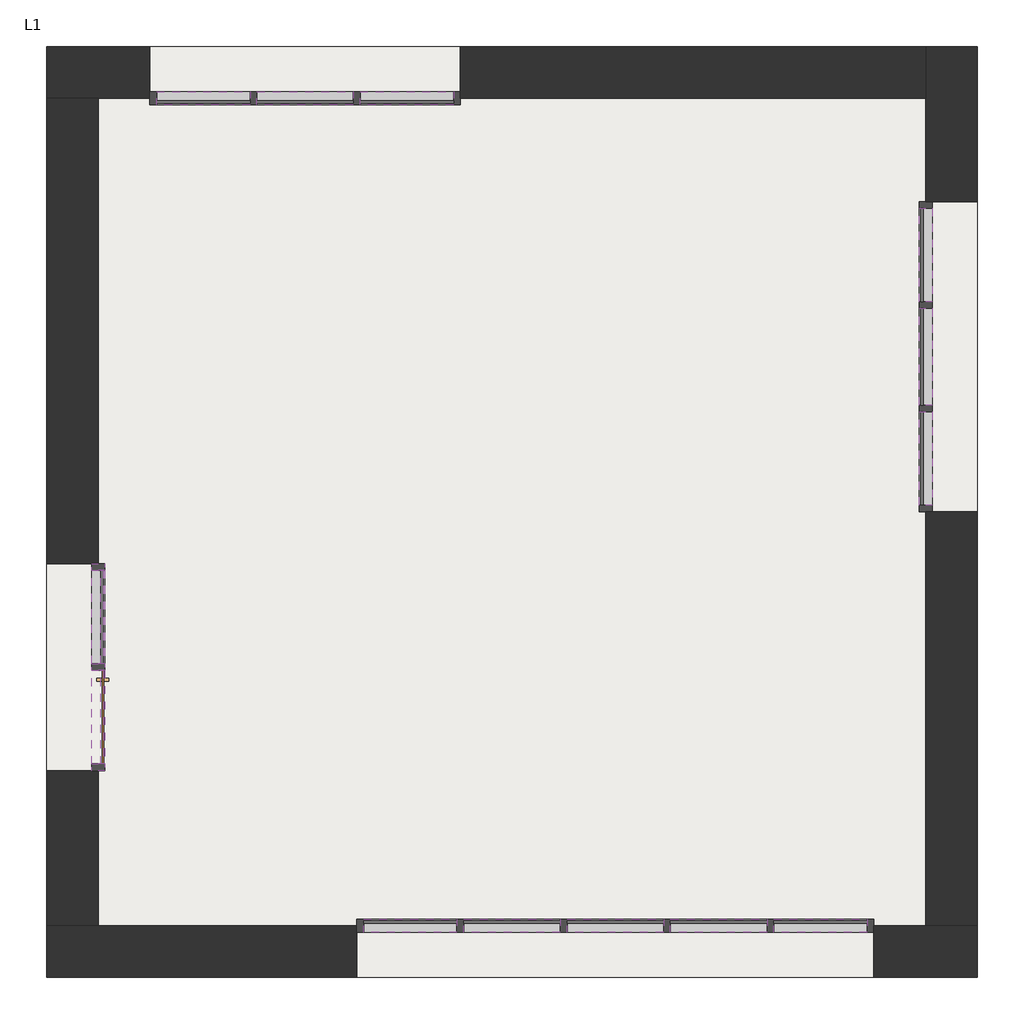
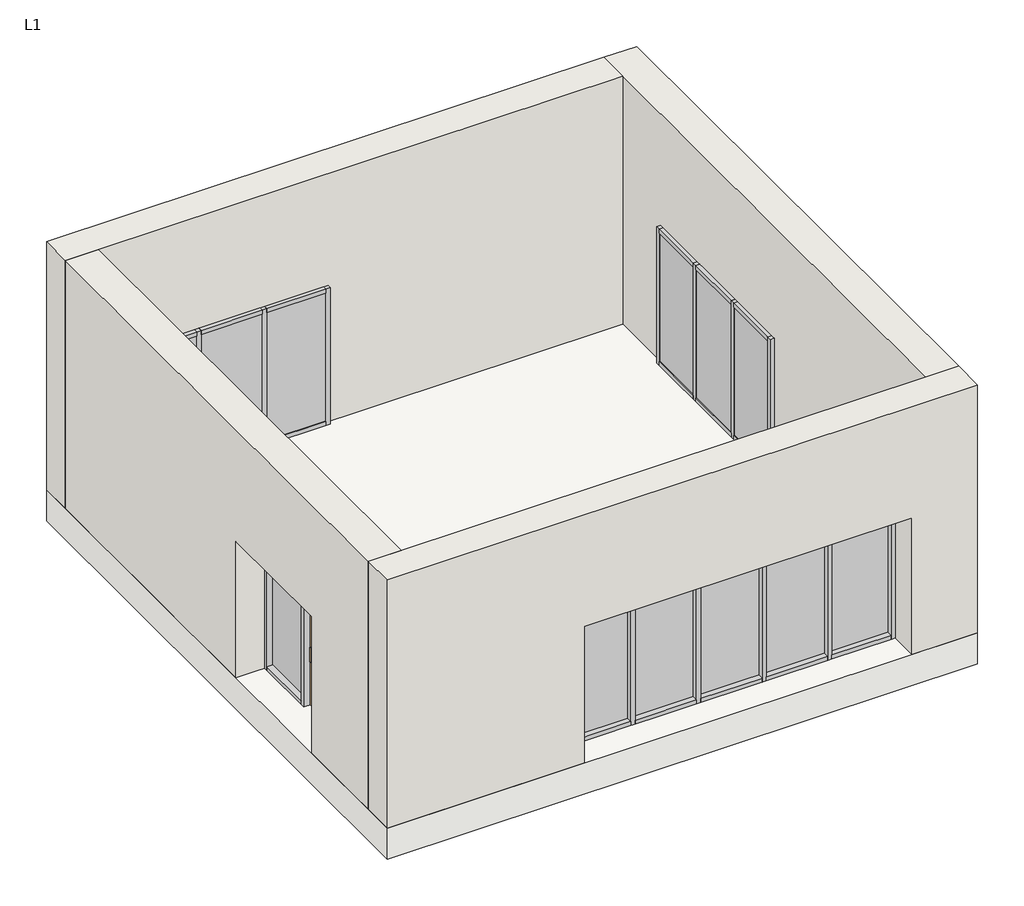
# One storey: 47 members, 14 plates, 4 walls, 1 door, 1 slab.
"""IFC4 building model written with IfcOpenShell, lengths in millimetres."""

import ifcopenshell
import ifcopenshell.guid

model = None  # the IFC model being written
_history = None  # IfcOwnerHistory: only IFC2X3 demands one
_inside = {}  # id of a spatial element -> (the spatial element, [elements in it])
_under = {}  # id of a project, library or spatial element -> (it, [spatial elements below it])
_declared = {}  # id of a project -> (the project, [libraries it declares])
_typed = {}  # id of a type object -> (the type object, [elements of that type])
_made_of = {}  # id of a material, layer set ... -> (it, [elements and type objects made of it])


def new_model(schema):
    """Start an empty IFC model of exactly this schema.

    Asked for "IFC4X3", IfcOpenShell would pick the latest addendum, in which some entities
    have other attributes; the version numbers below select the first issue.
    IFC2X3 requires an IfcOwnerHistory on every rooted entity: one is made here for all.
    """
    global model, _history
    if schema == "IFC4X3":
        model = ifcopenshell.file(schema_version=(4, 3, 0, 0))
    else:
        model = ifcopenshell.file(schema=schema)
    _inside.clear()
    _under.clear()
    _declared.clear()
    _typed.clear()
    _made_of.clear()
    _history = None
    if model.schema == "IFC2X3":
        org = make("IfcOrganization", Name="unknown")
        user = make(
            "IfcPersonAndOrganization",
            ThePerson=make("IfcPerson", FamilyName="unknown"),
            TheOrganization=org,
        )
        app = make(
            "IfcApplication",
            ApplicationDeveloper=org,
            Version="unknown",
            ApplicationFullName="unknown",
            ApplicationIdentifier="unknown",
        )
        _history = make(
            "IfcOwnerHistory",
            OwningUser=user,
            OwningApplication=app,
            ChangeAction="ADDED",
            CreationDate=0,
        )
    return model


def make(cls, **values):
    """One entity of the class cls with the attributes given. An attribute that is None is left unset."""
    return model.create_entity(
        cls, **{name: value for name, value in values.items() if value is not None}
    )


def rooted(cls, **values):
    """An entity with a GlobalId (a new one), such as an element, a storey or a relation."""
    return make(cls, GlobalId=ifcopenshell.guid.new(), OwnerHistory=_history, **values)


def si_unit(unit_type, name, prefix=None):
    """IfcSIUnit, for example si_unit("LENGTHUNIT", "METRE", prefix="MILLI")."""
    return make("IfcSIUnit", UnitType=unit_type, Prefix=prefix, Name=name)


def assignment(units):
    """IfcUnitAssignment: the units of a project."""
    return None if units is None else make("IfcUnitAssignment", Units=units)


def point(xyz):
    """IfcCartesianPoint."""
    return None if xyz is None else make("IfcCartesianPoint", Coordinates=xyz)


def direction(xyz):
    """IfcDirection."""
    return None if xyz is None else make("IfcDirection", DirectionRatios=xyz)


def frame(location, z_axis=None, x_axis=None):
    """IfcAxis2Placement3D, a coordinate frame: its origin and axes. An axis left out is left unset."""
    return make(
        "IfcAxis2Placement3D",
        Location=point(location),
        Axis=direction(z_axis),
        RefDirection=direction(x_axis),
    )


def origin():
    """The frame at (0, 0, 0) with its axes left unset."""
    return frame((0.0, 0.0, 0.0))


def origin_with_axes():
    """The frame at (0, 0, 0) with the z axis (0, 0, 1) and the x axis (1, 0, 0) written out."""
    return frame((0.0, 0.0, 0.0), z_axis=(0.0, 0.0, 1.0), x_axis=(1.0, 0.0, 0.0))


def place(relative_to, where):
    """IfcLocalPlacement: puts the frame where relative to a parent placement (None: the world)."""
    return make(
        "IfcLocalPlacement", PlacementRelTo=relative_to, RelativePlacement=where
    )


def context(
    kind, dimensions, precision=None, world=None, true_north=None, identifier=None
):
    """IfcGeometricRepresentationContext, for example the 3D "Model" context."""
    return make(
        "IfcGeometricRepresentationContext",
        ContextIdentifier=identifier,
        ContextType=kind,
        CoordinateSpaceDimension=dimensions,
        Precision=precision,
        WorldCoordinateSystem=world,
        TrueNorth=true_north,
    )


def project(units=None, contexts=None):
    """IfcProject with its units and contexts."""
    return rooted(
        "IfcProject",
        Name="project",
        RepresentationContexts=contexts,
        UnitsInContext=assignment(units),
    )


def spatial(cls, under=None, at=None, **own):
    """A site, building, storey or space (cls), placed at a placement, below another one or the project."""
    s = rooted(cls, ObjectPlacement=at, **own)
    if under is not None:
        _under.setdefault(under.id(), (under, []))[1].append(s)
    return s


def polyline(points):
    """IfcPolyline through the points."""
    return make("IfcPolyline", Points=[point(p) for p in points])


def outline(outer, holes=None, kind="AREA"):
    """IfcArbitraryClosedProfileDef: a profile drawn as a closed curve; with holes, ...WithVoids."""
    if holes is None:
        return make("IfcArbitraryClosedProfileDef", ProfileType=kind, OuterCurve=outer)
    return make(
        "IfcArbitraryProfileDefWithVoids",
        ProfileType=kind,
        OuterCurve=outer,
        InnerCurves=holes,
    )


def extrude(swept, where, along, depth):
    """IfcExtrudedAreaSolid: the profile swept, set in the frame where, extruded along a direction by depth."""
    return make(
        "IfcExtrudedAreaSolid",
        SweptArea=swept,
        Position=where,
        ExtrudedDirection=direction(along),
        Depth=depth,
    )


def faces_of(points, faces, orient=None, outer=None):
    """IfcFace entities. A face is a list of loops; a loop is a list of indices into points, from 0.

    orient and outer hold one flag for each loop. By default every Orientation is true, the
    first loop of a face is its IfcFaceOuterBound and the others are IfcFaceBound.
    """
    made = []
    for i, loops in enumerate(faces):
        bounds = []
        for j, loop in enumerate(loops):
            is_outer = j == 0 if outer is None else outer[i][j]
            bounds.append(
                make(
                    "IfcFaceOuterBound" if is_outer else "IfcFaceBound",
                    Bound=make("IfcPolyLoop", Polygon=[points[k] for k in loop]),
                    Orientation=True if orient is None else orient[i][j],
                )
            )
        made.append(make("IfcFace", Bounds=bounds))
    return made


def faceted_brep(points, faces, orient=None, outer=None, voids=None):
    """IfcFacetedBrep: a solid bounded by flat faces; with voids (closed shells), ...WithVoids."""
    shared = [point(p) for p in points]
    hull = make("IfcClosedShell", CfsFaces=faces_of(shared, faces, orient, outer))
    if voids is None:
        return make("IfcFacetedBrep", Outer=hull)
    return make(
        "IfcFacetedBrepWithVoids",
        Outer=hull,
        Voids=[
            make(cls, CfsFaces=faces_of(shared, fs, o, b)) for cls, fs, o, b in voids
        ],
    )


def shape(context_of_items, identifier, shape_type, items):
    """IfcShapeRepresentation: the items that make up one representation, for example the "Body"."""
    return make(
        "IfcShapeRepresentation",
        ContextOfItems=context_of_items,
        RepresentationIdentifier=identifier,
        RepresentationType=shape_type,
        Items=items,
    )


def source(mapping_origin, context_of_items, identifier, shape_type, items):
    """IfcRepresentationMap: a shape defined once, which mapped items show again and again."""
    return make(
        "IfcRepresentationMap",
        MappingOrigin=mapping_origin,
        MappedRepresentation=shape(context_of_items, identifier, shape_type, items),
    )


def transform(
    local_origin,
    x_axis=None,
    y_axis=None,
    z_axis=None,
    scale=None,
    scale2=None,
    scale3=None,
    uniform=True,
):
    """IfcCartesianTransformationOperator3D, or its non-uniform kind. x_axis, y_axis, z_axis: its Axis1, 2, 3."""
    if uniform:
        return make(
            "IfcCartesianTransformationOperator3D",
            Axis1=direction(x_axis),
            Axis2=direction(y_axis),
            LocalOrigin=point(local_origin),
            Scale=scale,
            Axis3=direction(z_axis),
        )
    return make(
        "IfcCartesianTransformationOperator3DnonUniform",
        Axis1=direction(x_axis),
        Axis2=direction(y_axis),
        LocalOrigin=point(local_origin),
        Scale=scale,
        Axis3=direction(z_axis),
        Scale2=scale2,
        Scale3=scale3,
    )


def mapped(mapping_source, mapping_target):
    """IfcMappedItem: shows the shape of a source again, moved by a transform."""
    return make(
        "IfcMappedItem", MappingSource=mapping_source, MappingTarget=mapping_target
    )


def made_of(thing, what):
    """Note that an element or type object is made of a material, layer set ...; save() writes the relation."""
    if what is not None:
        _made_of.setdefault(what.id(), (what, []))[1].append(thing)
    return thing


def element(
    cls,
    number,
    at=None,
    inside=None,
    cuts=None,
    type_object=None,
    material=None,
    context=None,
    identifier="Body",
    shape_type=None,
    held_by="IfcProductDefinitionShape",
    body=None,
    shapes=None,
    **own,
):
    """One element of the class cls, such as IfcWall. Its Tag is "e" and its number.

    at: its placement. inside: the storey or other place that contains it. cuts: it is an
    opening in that element (IfcRelVoidsElement). A single representation is given by context,
    identifier, shape_type and body (its items); several are given by shapes. held_by: the class
    of the entity that holds the representations. save() writes the other relations.
    """
    e = rooted(cls, Tag="e%d" % number, ObjectPlacement=at, **own)
    if body is not None:
        shapes = [shape(context, identifier, shape_type, body)]
    if shapes is not None:
        e.Representation = make(held_by, Representations=shapes)
    if inside is not None:
        _inside.setdefault(inside.id(), (inside, []))[1].append(e)
    if cuts is not None:
        rooted(
            "IfcRelVoidsElement", RelatingBuildingElement=cuts, RelatedOpeningElement=e
        )
    if type_object is not None:
        _typed.setdefault(type_object.id(), (type_object, []))[1].append(e)
    return made_of(e, material)


def aggregate(whole, parts):
    """IfcRelAggregates: a whole, such as a stair, and the parts it consists of."""
    return rooted("IfcRelAggregates", RelatingObject=whole, RelatedObjects=parts)


def save(model, path):
    """Write the relations noted so far, then the file.

    IfcRelAggregates (storeys below a building ...), IfcRelContainedInSpatialStructure (elements
    in a storey), IfcRelDefinesByType, IfcRelAssociatesMaterial and IfcRelDeclares: one each for
    every whole, place, type object, material and project.
    """
    for whole, parts in _under.values():
        aggregate(whole, parts)
    for where, things in _inside.values():
        rooted(
            "IfcRelContainedInSpatialStructure",
            RelatedElements=things,
            RelatingStructure=where,
        )
    for kind, things in _typed.values():
        rooted("IfcRelDefinesByType", RelatedObjects=things, RelatingType=kind)
    for what, things in _made_of.values():
        rooted("IfcRelAssociatesMaterial", RelatedObjects=things, RelatingMaterial=what)
    for by, libraries in _declared.values():
        rooted("IfcRelDeclares", RelatingContext=by, RelatedDefinitions=libraries)
    model.write(path)


def m_door_curtain_wall_single_glass_m_door_curtain_wall_single_b3f25844(model_context):
    return source(origin(), model_context, "Body", "SweptSolid", [
        extrude(outline(polyline([(451.2499998, 50.8), (451.2499998, 38.1), (-451.2499998, 38.1), (-451.2499998, 50.8), (451.2499998, 50.8)])), origin_with_axes(), (0.0, 0.0, 1.0), 1967.5),
        extrude(outline(polyline([(-375.0499998, 101.6), (-349.6499998, 101.6), (-349.6499998, 50.8), (-375.0499998, 50.8), (-375.0499998, 101.6)])), frame((0.0, 0.0, 762.0), z_axis=(0.0, 0.0, 1.0), x_axis=(1.0, 0.0, 0.0)), (0.0, 0.0, 1.0), 228.6),
        extrude(outline(polyline([(-349.6499998, -12.7), (-375.0499998, -12.7), (-375.0499998, 38.1), (-349.6499998, 38.1), (-349.6499998, -12.7)])), frame((0.0, 0.0, 762.0), z_axis=(0.0, 0.0, 1.0), x_axis=(1.0, 0.0, 0.0)), (0.0, 0.0, 1.0), 228.6),
    ])


def rectangular_mullion_65_x_125mm_rectangular_3ebb1efe(model_context):
    return source(origin(), model_context, "Body", "SweptSolid", [
        extrude(outline(polyline([(32.5, 62.5), (32.5, -62.5), (-32.5, -62.5), (-32.5, 62.5), (32.5, 62.5)])), frame((0.0, 0.0, -2200.0), z_axis=(0.0, 0.0, 1.0), x_axis=(1.0, 0.0, 0.0)), (0.0, 0.0, 1.0), 2200.0),
    ])


def rectangular_mullion_65_x_125mm_rectangular_02dc2359(model_context):
    return source(origin(), model_context, "Body", "SweptSolid", [
        extrude(outline(polyline([(0.0, 62.5), (0.0, -62.5), (-65.0, -62.5), (-65.0, 62.5), (0.0, 62.5)])), frame((0.0, 0.0, -2200.0), z_axis=(0.0, 0.0, 1.0), x_axis=(1.0, 0.0, 0.0)), (0.0, 0.0, 1.0), 2200.0),
    ])


def rectangular_mullion_65_x_125mm_rectangular_9a77bebc(model_context):
    return source(origin(), model_context, "Body", "SweptSolid", [
        extrude(outline(polyline([(0.0, 62.5), (0.0, -62.5), (-65.0, -62.5), (-65.0, 62.5), (0.0, 62.5)])), frame((0.0, 0.0, -902.5000003), z_axis=(0.0, 0.0, 1.0), x_axis=(1.0, 0.0, 0.0)), (0.0, 0.0, 1.0), 902.5000003),
    ])


def rectangular_mullion_65_x_125mm_rectangular_1b57746c(model_context):
    return source(origin(), model_context, "Body", "SweptSolid", [
        extrude(outline(polyline([(0.0, 62.5), (0.0, -62.5), (-65.0, -62.5), (-65.0, 62.5), (0.0, 62.5)])), frame((0.0, 0.0, -935.0), z_axis=(0.0, 0.0, 1.0), x_axis=(1.0, 0.0, 0.0)), (0.0, 0.0, 1.0), 935.0),
    ])


def rectangular_mullion_65_x_125mm_rectangular_ad388592(model_context):
    return source(origin(), model_context, "Body", "SweptSolid", [
        extrude(outline(polyline([(32.5, 62.5), (32.5, -62.5), (-32.5, -62.5), (-32.5, 62.5), (32.5, 62.5)])), frame((0.0, 0.0, -902.5000003), z_axis=(0.0, 0.0, 1.0), x_axis=(1.0, 0.0, 0.0)), (0.0, 0.0, 1.0), 902.5000003),
    ])


def rectangular_mullion_65_x_125mm_rectangular_470365d3(model_context):
    return source(origin(), model_context, "Body", "SweptSolid", [
        extrude(outline(polyline([(32.5, 62.5), (32.5, -62.5), (-32.5, -62.5), (-32.5, 62.5), (32.5, 62.5)])), frame((0.0, 0.0, -200.0), z_axis=(0.0, 0.0, 1.0), x_axis=(1.0, 0.0, 0.0)), (0.0, 0.0, 1.0), 200.0),
    ])


def rectangular_mullion_65_x_125mm_rectangular_dd0f1ba9(model_context):
    return source(origin(), model_context, "Body", "SweptSolid", [
        extrude(outline(polyline([(0.0, 62.5), (0.0, -62.5), (-65.0, -62.5), (-65.0, 62.5), (0.0, 62.5)])), frame((0.0, 0.0, -200.0), z_axis=(0.0, 0.0, 1.0), x_axis=(1.0, 0.0, 0.0)), (0.0, 0.0, 1.0), 200.0),
    ])


def rectangular_mullion_65_x_125mm_rectangular_b62c991d(model_context):
    return source(origin(), model_context, "Body", "SweptSolid", [
        extrude(outline(polyline([(32.5, 62.5), (32.5, -62.5), (-32.5, -62.5), (-32.5, 62.5), (32.5, 62.5)])), frame((0.0, 0.0, -2000.0), z_axis=(0.0, 0.0, 1.0), x_axis=(1.0, 0.0, 0.0)), (0.0, 0.0, 1.0), 2000.0),
    ])


def rectangular_mullion_65_x_125mm_rectangular_d57ab73f(model_context):
    return source(origin(), model_context, "Body", "SweptSolid", [
        extrude(outline(polyline([(0.0, 62.5), (0.0, -62.5), (-65.0, -62.5), (-65.0, 62.5), (0.0, 62.5)])), frame((0.0, 0.0, -2000.0), z_axis=(0.0, 0.0, 1.0), x_axis=(1.0, 0.0, 0.0)), (0.0, 0.0, 1.0), 2000.0),
    ])


def system_panel_glazed_3f8cfcef(model_context):
    return source(origin(), model_context, "Body", "SweptSolid", [
        extrude(outline(polyline([(451.2500002, 24.5), (-451.2500002, 24.5), (-451.2500002, 49.5), (451.2500002, 49.5), (451.2500002, 24.5)])), origin_with_axes(), (0.0, 0.0, 1.0), 2070.0),
    ])


def system_panel_glazed_4c7b465e(model_context):
    return source(origin(), model_context, "Body", "SweptSolid", [
        extrude(outline(polyline([(467.5, 24.5), (-467.5, 24.5), (-467.5, 49.5), (467.5, 49.5), (467.5, 24.5)])), origin_with_axes(), (0.0, 0.0, 1.0), 2070.0),
    ])


def system_panel_glazed_7330a8e7(model_context):
    return source(origin(), model_context, "Body", "SweptSolid", [
        extrude(outline(polyline([(451.2500002, 24.5), (-451.2500002, 24.5), (-451.2500002, 49.5), (451.2500002, 49.5), (451.2500002, 24.5)])), origin_with_axes(), (0.0, 0.0, 1.0), 102.5),
    ])


def system_panel_glazed_53f32d20(model_context):
    return source(origin(), model_context, "Body", "SweptSolid", [
        extrude(outline(polyline([(451.2500002, 24.5), (-451.2500002, 24.5), (-451.2500002, 49.5), (451.2500002, 49.5), (451.2500002, 24.5)])), origin_with_axes(), (0.0, 0.0, 1.0), 1902.5),
    ])


model = new_model("IFC4")

# Units and contexts
model_context = context("Model", 3, world=origin())
ifc_project = project(units=[si_unit("LENGTHUNIT", "METRE", prefix="MILLI")], contexts=[model_context])

# Site, building, storey
site = spatial("IfcSite", under=ifc_project)
building = spatial("IfcBuilding", under=site)
storey = spatial("IfcBuildingStorey", under=building, Name="L1", Elevation=0.0)

# Door
placement = place(None, origin())
m_door_curtain_wall_single_glass_m_door_curtain_wall_single_shape = m_door_curtain_wall_single_glass_m_door_curtain_wall_single_b3f25844(model_context)
element("IfcDoor", 1, ObjectType="M_Door-Curtain-Wall-Single-Glass : M_Door-Curtain-Wall-Single-Glass", at=placement, inside=storey, context=model_context, shape_type="MappedRepresentation", body=[
    mapped(m_door_curtain_wall_single_glass_m_door_curtain_wall_single_shape, transform((500.000016, 1516.2441438, 0.0), x_axis=(0.0, -1.0, 0.0), y_axis=(1.0, 0.0, 0.0), z_axis=(0.0, 0.0, 1.0))),
])

# Members
rectangular_mullion_65_x_125mm_rectangular_shape = rectangular_mullion_65_x_125mm_rectangular_3ebb1efe(model_context)
element("IfcMember", 2, ObjectType="Rectangular Mullion : 65 x 125mm rectangular", at=placement, inside=storey, context=model_context, shape_type="MappedRepresentation", body=[
    mapped(rectangular_mullion_65_x_125mm_rectangular_shape, transform((4000.0000163, -500.0058491, 0.0), x_axis=(1.0, 0.0, 0.0), y_axis=(0.0, -1.0, 0.0), z_axis=(0.0, 0.0, -1.0))),
])
element("IfcMember", 3, ObjectType="Rectangular Mullion : 65 x 125mm rectangular", at=placement, inside=storey, context=model_context, shape_type="MappedRepresentation", body=[
    mapped(rectangular_mullion_65_x_125mm_rectangular_shape, transform((5000.0000163, -500.0058491, 0.0), x_axis=(1.0, 0.0, 0.0), y_axis=(0.0, -1.0, 0.0), z_axis=(0.0, 0.0, -1.0))),
])
element("IfcMember", 4, ObjectType="Rectangular Mullion : 65 x 125mm rectangular", at=placement, inside=storey, context=model_context, shape_type="MappedRepresentation", body=[
    mapped(rectangular_mullion_65_x_125mm_rectangular_shape, transform((6000.0000163, -500.0058491, 0.0), x_axis=(1.0, 0.0, 0.0), y_axis=(0.0, -1.0, 0.0), z_axis=(0.0, 0.0, -1.0))),
])
element("IfcMember", 5, ObjectType="Rectangular Mullion : 65 x 125mm rectangular", at=placement, inside=storey, context=model_context, shape_type="MappedRepresentation", body=[
    mapped(rectangular_mullion_65_x_125mm_rectangular_shape, transform((7000.0000163, -500.0058491, 0.0), x_axis=(1.0, 0.0, 0.0), y_axis=(0.0, -1.0, 0.0), z_axis=(0.0, 0.0, -1.0))),
])
element("IfcMember", 6, ObjectType="Rectangular Mullion : 65 x 125mm rectangular", at=placement, inside=storey, context=model_context, shape_type="MappedRepresentation", body=[
    mapped(rectangular_mullion_65_x_125mm_rectangular_shape, transform((8500.000016, 4499.9941443, 0.0), x_axis=(0.0, 1.0, 0.0), y_axis=(1.0, 0.0, 0.0), z_axis=(0.0, 0.0, -1.0))),
])
element("IfcMember", 7, ObjectType="Rectangular Mullion : 65 x 125mm rectangular", at=placement, inside=storey, context=model_context, shape_type="MappedRepresentation", body=[
    mapped(rectangular_mullion_65_x_125mm_rectangular_shape, transform((8500.000016, 5499.9941443, 0.0), x_axis=(0.0, 1.0, 0.0), y_axis=(1.0, 0.0, 0.0), z_axis=(0.0, 0.0, -1.0))),
])
element("IfcMember", 8, ObjectType="Rectangular Mullion : 65 x 125mm rectangular", at=placement, inside=storey, context=model_context, shape_type="MappedRepresentation", body=[
    mapped(rectangular_mullion_65_x_125mm_rectangular_shape, transform((3000.0000157, 7499.994144, 0.0), x_axis=(-1.0, 0.0, 0.0), y_axis=(0.0, 1.0, 0.0), z_axis=(0.0, 0.0, -1.0))),
])
element("IfcMember", 9, ObjectType="Rectangular Mullion : 65 x 125mm rectangular", at=placement, inside=storey, context=model_context, shape_type="MappedRepresentation", body=[
    mapped(rectangular_mullion_65_x_125mm_rectangular_shape, transform((2000.0000157, 7499.994144, 0.0), x_axis=(-1.0, 0.0, 0.0), y_axis=(0.0, 1.0, 0.0), z_axis=(0.0, 0.0, -1.0))),
])
rectangular_mullion_65_x_125mm_rectangular_2_shape = rectangular_mullion_65_x_125mm_rectangular_02dc2359(model_context)
element("IfcMember", 10, ObjectType="Rectangular Mullion : 65 x 125mm rectangular", at=placement, inside=storey, context=model_context, shape_type="MappedRepresentation", body=[
    mapped(rectangular_mullion_65_x_125mm_rectangular_2_shape, transform((8000.000016, -500.0058491, 0.0), x_axis=(1.0, 0.0, 0.0), y_axis=(0.0, -1.0, 0.0), z_axis=(0.0, 0.0, -1.0))),
])
element("IfcMember", 11, ObjectType="Rectangular Mullion : 65 x 125mm rectangular", at=placement, inside=storey, context=model_context, shape_type="MappedRepresentation", body=[
    mapped(rectangular_mullion_65_x_125mm_rectangular_2_shape, transform((8500.000016, 6499.994144, 0.0), x_axis=(0.0, 1.0, 0.0), y_axis=(1.0, 0.0, 0.0), z_axis=(0.0, 0.0, -1.0))),
])
element("IfcMember", 12, ObjectType="Rectangular Mullion : 65 x 125mm rectangular", at=placement, inside=storey, context=model_context, shape_type="MappedRepresentation", body=[
    mapped(rectangular_mullion_65_x_125mm_rectangular_2_shape, transform((1000.000016, 7499.994144, 0.0), x_axis=(-1.0, 0.0, 0.0), y_axis=(0.0, 1.0, 0.0), z_axis=(0.0, 0.0, -1.0))),
])
element("IfcMember", 13, ObjectType="Rectangular Mullion : 65 x 125mm rectangular", at=placement, inside=storey, context=model_context, shape_type="MappedRepresentation", body=[
    mapped(rectangular_mullion_65_x_125mm_rectangular_2_shape, transform((3000.000016, -500.0058491, 2200.0), x_axis=(-1.0, 0.0, 0.0), y_axis=(0.0, -1.0, 0.0), z_axis=(0.0, 0.0, 1.0))),
])
element("IfcMember", 14, ObjectType="Rectangular Mullion : 65 x 125mm rectangular", at=placement, inside=storey, context=model_context, shape_type="MappedRepresentation", body=[
    mapped(rectangular_mullion_65_x_125mm_rectangular_2_shape, transform((8500.000016, 3499.994144, 2200.0), x_axis=(0.0, -1.0, 0.0), y_axis=(1.0, 0.0, 0.0), z_axis=(0.0, 0.0, 1.0))),
])
element("IfcMember", 15, ObjectType="Rectangular Mullion : 65 x 125mm rectangular", at=placement, inside=storey, context=model_context, shape_type="MappedRepresentation", body=[
    mapped(rectangular_mullion_65_x_125mm_rectangular_2_shape, transform((4000.000016, 7499.994144, 2200.0), x_axis=(1.0, 0.0, 0.0), y_axis=(0.0, 1.0, 0.0), z_axis=(0.0, 0.0, 1.0))),
])
rectangular_mullion_65_x_125mm_rectangular_3_shape = rectangular_mullion_65_x_125mm_rectangular_9a77bebc(model_context)
element("IfcMember", 16, ObjectType="Rectangular Mullion : 65 x 125mm rectangular", at=placement, inside=storey, context=model_context, shape_type="MappedRepresentation", body=[
    mapped(rectangular_mullion_65_x_125mm_rectangular_3_shape, transform((7935.000016, -500.0058491, 2200.0), x_axis=(0.0, 0.0, 1.0), y_axis=(0.0, -1.0, 0.0), z_axis=(1.0, 0.0, 0.0))),
])
element("IfcMember", 17, ObjectType="Rectangular Mullion : 65 x 125mm rectangular", at=placement, inside=storey, context=model_context, shape_type="MappedRepresentation", body=[
    mapped(rectangular_mullion_65_x_125mm_rectangular_3_shape, transform((3967.5000163, -500.0058491, 2200.0), x_axis=(0.0, 0.0, 1.0), y_axis=(0.0, -1.0, 0.0), z_axis=(1.0, 0.0, 0.0))),
])
element("IfcMember", 18, ObjectType="Rectangular Mullion : 65 x 125mm rectangular", at=placement, inside=storey, context=model_context, shape_type="MappedRepresentation", body=[
    mapped(rectangular_mullion_65_x_125mm_rectangular_3_shape, transform((8500.000016, 6434.994144, 2200.0), x_axis=(0.0, 0.0, 1.0), y_axis=(1.0, 0.0, 0.0), z_axis=(0.0, 1.0, 0.0))),
])
element("IfcMember", 19, ObjectType="Rectangular Mullion : 65 x 125mm rectangular", at=placement, inside=storey, context=model_context, shape_type="MappedRepresentation", body=[
    mapped(rectangular_mullion_65_x_125mm_rectangular_3_shape, transform((8500.000016, 4467.4941443, 2200.0), x_axis=(0.0, 0.0, 1.0), y_axis=(1.0, 0.0, 0.0), z_axis=(0.0, 1.0, 0.0))),
])
element("IfcMember", 20, ObjectType="Rectangular Mullion : 65 x 125mm rectangular", at=placement, inside=storey, context=model_context, shape_type="MappedRepresentation", body=[
    mapped(rectangular_mullion_65_x_125mm_rectangular_3_shape, transform((1065.000016, 7499.994144, 2200.0), x_axis=(0.0, 0.0, 1.0), y_axis=(0.0, 1.0, 0.0), z_axis=(-1.0, 0.0, 0.0))),
])
element("IfcMember", 21, ObjectType="Rectangular Mullion : 65 x 125mm rectangular", at=placement, inside=storey, context=model_context, shape_type="MappedRepresentation", body=[
    mapped(rectangular_mullion_65_x_125mm_rectangular_3_shape, transform((3032.5000157, 7499.994144, 2200.0), x_axis=(0.0, 0.0, 1.0), y_axis=(0.0, 1.0, 0.0), z_axis=(-1.0, 0.0, 0.0))),
])
element("IfcMember", 22, ObjectType="Rectangular Mullion : 65 x 125mm rectangular", at=placement, inside=storey, context=model_context, shape_type="MappedRepresentation", body=[
    mapped(rectangular_mullion_65_x_125mm_rectangular_3_shape, transform((500.000016, 1064.994144, 2200.0), x_axis=(0.0, 0.0, 1.0), y_axis=(-1.0, 0.0, 0.0), z_axis=(0.0, -1.0, 0.0))),
])
element("IfcMember", 23, ObjectType="Rectangular Mullion : 65 x 125mm rectangular", at=placement, inside=storey, context=model_context, shape_type="MappedRepresentation", body=[
    mapped(rectangular_mullion_65_x_125mm_rectangular_3_shape, transform((500.000016, 2032.4941437, 2200.0), x_axis=(0.0, 0.0, 1.0), y_axis=(-1.0, 0.0, 0.0), z_axis=(0.0, -1.0, 0.0))),
])
rectangular_mullion_65_x_125mm_rectangular_4_shape = rectangular_mullion_65_x_125mm_rectangular_1b57746c(model_context)
element("IfcMember", 24, ObjectType="Rectangular Mullion : 65 x 125mm rectangular", at=placement, inside=storey, context=model_context, shape_type="MappedRepresentation", body=[
    mapped(rectangular_mullion_65_x_125mm_rectangular_4_shape, transform((4967.5000163, -500.0058491, 2200.0), x_axis=(0.0, 0.0, 1.0), y_axis=(0.0, -1.0, 0.0), z_axis=(1.0, 0.0, 0.0))),
])
element("IfcMember", 25, ObjectType="Rectangular Mullion : 65 x 125mm rectangular", at=placement, inside=storey, context=model_context, shape_type="MappedRepresentation", body=[
    mapped(rectangular_mullion_65_x_125mm_rectangular_4_shape, transform((5967.5000163, -500.0058491, 2200.0), x_axis=(0.0, 0.0, 1.0), y_axis=(0.0, -1.0, 0.0), z_axis=(1.0, 0.0, 0.0))),
])
element("IfcMember", 26, ObjectType="Rectangular Mullion : 65 x 125mm rectangular", at=placement, inside=storey, context=model_context, shape_type="MappedRepresentation", body=[
    mapped(rectangular_mullion_65_x_125mm_rectangular_4_shape, transform((6967.5000163, -500.0058491, 2200.0), x_axis=(0.0, 0.0, 1.0), y_axis=(0.0, -1.0, 0.0), z_axis=(1.0, 0.0, 0.0))),
])
element("IfcMember", 27, ObjectType="Rectangular Mullion : 65 x 125mm rectangular", at=placement, inside=storey, context=model_context, shape_type="MappedRepresentation", body=[
    mapped(rectangular_mullion_65_x_125mm_rectangular_4_shape, transform((8500.000016, 5467.4941443, 2200.0), x_axis=(0.0, 0.0, 1.0), y_axis=(1.0, 0.0, 0.0), z_axis=(0.0, 1.0, 0.0))),
])
element("IfcMember", 28, ObjectType="Rectangular Mullion : 65 x 125mm rectangular", at=placement, inside=storey, context=model_context, shape_type="MappedRepresentation", body=[
    mapped(rectangular_mullion_65_x_125mm_rectangular_4_shape, transform((2032.5000157, 7499.994144, 2200.0), x_axis=(0.0, 0.0, 1.0), y_axis=(0.0, 1.0, 0.0), z_axis=(-1.0, 0.0, 0.0))),
])
element("IfcMember", 29, ObjectType="Rectangular Mullion : 65 x 125mm rectangular", at=placement, inside=storey, context=model_context, shape_type="MappedRepresentation", body=[
    mapped(rectangular_mullion_65_x_125mm_rectangular_3_shape, transform((3065.000016, -500.0058491, 0.0), x_axis=(0.0, 0.0, -1.0), y_axis=(0.0, -1.0, 0.0), z_axis=(-1.0, 0.0, 0.0))),
])
element("IfcMember", 30, ObjectType="Rectangular Mullion : 65 x 125mm rectangular", at=placement, inside=storey, context=model_context, shape_type="MappedRepresentation", body=[
    mapped(rectangular_mullion_65_x_125mm_rectangular_3_shape, transform((7032.5000163, -500.0058491, 0.0), x_axis=(0.0, 0.0, -1.0), y_axis=(0.0, -1.0, 0.0), z_axis=(-1.0, 0.0, 0.0))),
])
element("IfcMember", 31, ObjectType="Rectangular Mullion : 65 x 125mm rectangular", at=placement, inside=storey, context=model_context, shape_type="MappedRepresentation", body=[
    mapped(rectangular_mullion_65_x_125mm_rectangular_3_shape, transform((8500.000016, 3564.994144, 0.0), x_axis=(0.0, 0.0, -1.0), y_axis=(1.0, 0.0, 0.0), z_axis=(0.0, -1.0, 0.0))),
])
element("IfcMember", 32, ObjectType="Rectangular Mullion : 65 x 125mm rectangular", at=placement, inside=storey, context=model_context, shape_type="MappedRepresentation", body=[
    mapped(rectangular_mullion_65_x_125mm_rectangular_3_shape, transform((8500.000016, 5532.4941443, 0.0), x_axis=(0.0, 0.0, -1.0), y_axis=(1.0, 0.0, 0.0), z_axis=(0.0, -1.0, 0.0))),
])
element("IfcMember", 33, ObjectType="Rectangular Mullion : 65 x 125mm rectangular", at=placement, inside=storey, context=model_context, shape_type="MappedRepresentation", body=[
    mapped(rectangular_mullion_65_x_125mm_rectangular_3_shape, transform((3935.000016, 7499.994144, 0.0), x_axis=(0.0, 0.0, -1.0), y_axis=(0.0, 1.0, 0.0), z_axis=(1.0, 0.0, 0.0))),
])
element("IfcMember", 34, ObjectType="Rectangular Mullion : 65 x 125mm rectangular", at=placement, inside=storey, context=model_context, shape_type="MappedRepresentation", body=[
    mapped(rectangular_mullion_65_x_125mm_rectangular_3_shape, transform((1967.5000157, 7499.994144, 0.0), x_axis=(0.0, 0.0, -1.0), y_axis=(0.0, 1.0, 0.0), z_axis=(1.0, 0.0, 0.0))),
])
element("IfcMember", 35, ObjectType="Rectangular Mullion : 65 x 125mm rectangular", at=placement, inside=storey, context=model_context, shape_type="MappedRepresentation", body=[
    mapped(rectangular_mullion_65_x_125mm_rectangular_3_shape, transform((500.000016, 2934.994144, 0.0), x_axis=(0.0, 0.0, -1.0), y_axis=(-1.0, 0.0, 0.0), z_axis=(0.0, 1.0, 0.0))),
])
element("IfcMember", 36, ObjectType="Rectangular Mullion : 65 x 125mm rectangular", at=placement, inside=storey, context=model_context, shape_type="MappedRepresentation", body=[
    mapped(rectangular_mullion_65_x_125mm_rectangular_4_shape, transform((4032.5000163, -500.0058491, 0.0), x_axis=(0.0, 0.0, -1.0), y_axis=(0.0, -1.0, 0.0), z_axis=(-1.0, 0.0, 0.0))),
])
element("IfcMember", 37, ObjectType="Rectangular Mullion : 65 x 125mm rectangular", at=placement, inside=storey, context=model_context, shape_type="MappedRepresentation", body=[
    mapped(rectangular_mullion_65_x_125mm_rectangular_4_shape, transform((5032.5000163, -500.0058491, 0.0), x_axis=(0.0, 0.0, -1.0), y_axis=(0.0, -1.0, 0.0), z_axis=(-1.0, 0.0, 0.0))),
])
element("IfcMember", 38, ObjectType="Rectangular Mullion : 65 x 125mm rectangular", at=placement, inside=storey, context=model_context, shape_type="MappedRepresentation", body=[
    mapped(rectangular_mullion_65_x_125mm_rectangular_4_shape, transform((6032.5000163, -500.0058491, 0.0), x_axis=(0.0, 0.0, -1.0), y_axis=(0.0, -1.0, 0.0), z_axis=(-1.0, 0.0, 0.0))),
])
element("IfcMember", 39, ObjectType="Rectangular Mullion : 65 x 125mm rectangular", at=placement, inside=storey, context=model_context, shape_type="MappedRepresentation", body=[
    mapped(rectangular_mullion_65_x_125mm_rectangular_4_shape, transform((8500.000016, 4532.4941443, 0.0), x_axis=(0.0, 0.0, -1.0), y_axis=(1.0, 0.0, 0.0), z_axis=(0.0, -1.0, 0.0))),
])
element("IfcMember", 40, ObjectType="Rectangular Mullion : 65 x 125mm rectangular", at=placement, inside=storey, context=model_context, shape_type="MappedRepresentation", body=[
    mapped(rectangular_mullion_65_x_125mm_rectangular_4_shape, transform((2967.5000157, 7499.994144, 0.0), x_axis=(0.0, 0.0, -1.0), y_axis=(0.0, 1.0, 0.0), z_axis=(1.0, 0.0, 0.0))),
])
rectangular_mullion_65_x_125mm_rectangular_5_shape = rectangular_mullion_65_x_125mm_rectangular_ad388592(model_context)
element("IfcMember", 41, ObjectType="Rectangular Mullion : 65 x 125mm rectangular", at=placement, inside=storey, context=model_context, shape_type="MappedRepresentation", body=[
    mapped(rectangular_mullion_65_x_125mm_rectangular_5_shape, transform((500.000016, 2032.4941437, 2000.0), x_axis=(0.0, 0.0, 1.0), y_axis=(-1.0, 0.0, 0.0), z_axis=(0.0, -1.0, 0.0))),
])
element("IfcMember", 42, ObjectType="Rectangular Mullion : 65 x 125mm rectangular", at=placement, inside=storey, context=model_context, shape_type="MappedRepresentation", body=[
    mapped(rectangular_mullion_65_x_125mm_rectangular_5_shape, transform((500.000016, 1064.994144, 2000.0), x_axis=(0.0, 0.0, 1.0), y_axis=(-1.0, 0.0, 0.0), z_axis=(0.0, -1.0, 0.0))),
])
rectangular_mullion_65_x_125mm_rectangular_6_shape = rectangular_mullion_65_x_125mm_rectangular_470365d3(model_context)
element("IfcMember", 43, ObjectType="Rectangular Mullion : 65 x 125mm rectangular", at=placement, inside=storey, context=model_context, shape_type="MappedRepresentation", body=[
    mapped(rectangular_mullion_65_x_125mm_rectangular_6_shape, transform((500.000016, 1999.9941437, 2000.0), x_axis=(0.0, -1.0, 0.0), y_axis=(-1.0, 0.0, 0.0), z_axis=(0.0, 0.0, -1.0))),
])
rectangular_mullion_65_x_125mm_rectangular_7_shape = rectangular_mullion_65_x_125mm_rectangular_dd0f1ba9(model_context)
element("IfcMember", 44, ObjectType="Rectangular Mullion : 65 x 125mm rectangular", at=placement, inside=storey, context=model_context, shape_type="MappedRepresentation", body=[
    mapped(rectangular_mullion_65_x_125mm_rectangular_7_shape, transform((500.000016, 999.994144, 2000.0), x_axis=(0.0, -1.0, 0.0), y_axis=(-1.0, 0.0, 0.0), z_axis=(0.0, 0.0, -1.0))),
])
element("IfcMember", 45, ObjectType="Rectangular Mullion : 65 x 125mm rectangular", at=placement, inside=storey, context=model_context, shape_type="MappedRepresentation", body=[
    mapped(rectangular_mullion_65_x_125mm_rectangular_7_shape, transform((500.000016, 2999.994144, 2200.0), x_axis=(0.0, 1.0, 0.0), y_axis=(-1.0, 0.0, 0.0), z_axis=(0.0, 0.0, 1.0))),
])
rectangular_mullion_65_x_125mm_rectangular_8_shape = rectangular_mullion_65_x_125mm_rectangular_b62c991d(model_context)
element("IfcMember", 46, ObjectType="Rectangular Mullion : 65 x 125mm rectangular", at=placement, inside=storey, context=model_context, shape_type="MappedRepresentation", body=[
    mapped(rectangular_mullion_65_x_125mm_rectangular_8_shape, transform((500.000016, 1999.9941437, 0.0), x_axis=(0.0, -1.0, 0.0), y_axis=(-1.0, 0.0, 0.0), z_axis=(0.0, 0.0, -1.0))),
])
rectangular_mullion_65_x_125mm_rectangular_9_shape = rectangular_mullion_65_x_125mm_rectangular_d57ab73f(model_context)
element("IfcMember", 47, ObjectType="Rectangular Mullion : 65 x 125mm rectangular", at=placement, inside=storey, context=model_context, shape_type="MappedRepresentation", body=[
    mapped(rectangular_mullion_65_x_125mm_rectangular_9_shape, transform((500.000016, 2999.994144, 2000.0), x_axis=(0.0, 1.0, 0.0), y_axis=(-1.0, 0.0, 0.0), z_axis=(0.0, 0.0, 1.0))),
])
element("IfcMember", 48, ObjectType="Rectangular Mullion : 65 x 125mm rectangular", at=placement, inside=storey, context=model_context, shape_type="MappedRepresentation", body=[
    mapped(rectangular_mullion_65_x_125mm_rectangular_9_shape, transform((500.000016, 999.994144, 0.0), x_axis=(0.0, -1.0, 0.0), y_axis=(-1.0, 0.0, 0.0), z_axis=(0.0, 0.0, -1.0))),
])

# Plates
system_panel_glazed_shape = system_panel_glazed_3f8cfcef(model_context)
element("IfcPlate", 49, ObjectType="System Panel : Glazed", at=placement, inside=storey, context=model_context, shape_type="MappedRepresentation", body=[
    mapped(system_panel_glazed_shape, transform((3516.2500162, -500.0058491, 65.0), x_axis=(1.0, 0.0, 0.0), y_axis=(0.0, 1.0, 0.0), z_axis=(0.0, 0.0, 1.0))),
])
element("IfcPlate", 50, ObjectType="System Panel : Glazed", at=placement, inside=storey, context=model_context, shape_type="MappedRepresentation", body=[
    mapped(system_panel_glazed_shape, transform((7483.7500162, -500.0058491, 65.0), x_axis=(1.0, 0.0, 0.0), y_axis=(0.0, 1.0, 0.0), z_axis=(0.0, 0.0, 1.0))),
])
element("IfcPlate", 51, ObjectType="System Panel : Glazed", at=placement, inside=storey, context=model_context, shape_type="MappedRepresentation", body=[
    mapped(system_panel_glazed_shape, transform((8500.000016, 4016.2441442, 65.0), x_axis=(0.0, 1.0, 0.0), y_axis=(-1.0, 0.0, 0.0), z_axis=(0.0, 0.0, 1.0))),
])
element("IfcPlate", 52, ObjectType="System Panel : Glazed", at=placement, inside=storey, context=model_context, shape_type="MappedRepresentation", body=[
    mapped(system_panel_glazed_shape, transform((8500.000016, 5983.7441442, 65.0), x_axis=(0.0, 1.0, 0.0), y_axis=(-1.0, 0.0, 0.0), z_axis=(0.0, 0.0, 1.0))),
])
element("IfcPlate", 53, ObjectType="System Panel : Glazed", at=placement, inside=storey, context=model_context, shape_type="MappedRepresentation", body=[
    mapped(system_panel_glazed_shape, transform((3483.7500158, 7499.994144, 65.0), x_axis=(-1.0, 0.0, 0.0), y_axis=(0.0, -1.0, 0.0), z_axis=(0.0, 0.0, 1.0))),
])
element("IfcPlate", 54, ObjectType="System Panel : Glazed", at=placement, inside=storey, context=model_context, shape_type="MappedRepresentation", body=[
    mapped(system_panel_glazed_shape, transform((1516.2500158, 7499.994144, 65.0), x_axis=(-1.0, 0.0, 0.0), y_axis=(0.0, -1.0, 0.0), z_axis=(0.0, 0.0, 1.0))),
])
system_panel_glazed_2_shape = system_panel_glazed_4c7b465e(model_context)
element("IfcPlate", 55, ObjectType="System Panel : Glazed", at=placement, inside=storey, context=model_context, shape_type="MappedRepresentation", body=[
    mapped(system_panel_glazed_2_shape, transform((4500.0000163, -500.0058491, 65.0), x_axis=(1.0, 0.0, 0.0), y_axis=(0.0, 1.0, 0.0), z_axis=(0.0, 0.0, 1.0))),
])
element("IfcPlate", 56, ObjectType="System Panel : Glazed", at=placement, inside=storey, context=model_context, shape_type="MappedRepresentation", body=[
    mapped(system_panel_glazed_2_shape, transform((5500.0000163, -500.0058491, 65.0), x_axis=(1.0, 0.0, 0.0), y_axis=(0.0, 1.0, 0.0), z_axis=(0.0, 0.0, 1.0))),
])
element("IfcPlate", 57, ObjectType="System Panel : Glazed", at=placement, inside=storey, context=model_context, shape_type="MappedRepresentation", body=[
    mapped(system_panel_glazed_2_shape, transform((6500.0000163, -500.0058491, 65.0), x_axis=(1.0, 0.0, 0.0), y_axis=(0.0, 1.0, 0.0), z_axis=(0.0, 0.0, 1.0))),
])
element("IfcPlate", 58, ObjectType="System Panel : Glazed", at=placement, inside=storey, context=model_context, shape_type="MappedRepresentation", body=[
    mapped(system_panel_glazed_2_shape, transform((8500.000016, 4999.9941443, 65.0), x_axis=(0.0, 1.0, 0.0), y_axis=(-1.0, 0.0, 0.0), z_axis=(0.0, 0.0, 1.0))),
])
element("IfcPlate", 59, ObjectType="System Panel : Glazed", at=placement, inside=storey, context=model_context, shape_type="MappedRepresentation", body=[
    mapped(system_panel_glazed_2_shape, transform((2500.0000157, 7499.994144, 65.0), x_axis=(-1.0, 0.0, 0.0), y_axis=(0.0, -1.0, 0.0), z_axis=(0.0, 0.0, 1.0))),
])
system_panel_glazed_3_shape = system_panel_glazed_7330a8e7(model_context)
element("IfcPlate", 60, ObjectType="System Panel : Glazed", at=placement, inside=storey, context=model_context, shape_type="MappedRepresentation", body=[
    mapped(system_panel_glazed_3_shape, transform((500.000016, 2483.7441438, 2032.5), x_axis=(0.0, -1.0, 0.0), y_axis=(1.0, 0.0, 0.0), z_axis=(0.0, 0.0, 1.0))),
])
element("IfcPlate", 61, ObjectType="System Panel : Glazed", at=placement, inside=storey, context=model_context, shape_type="MappedRepresentation", body=[
    mapped(system_panel_glazed_3_shape, transform((500.000016, 1516.2441438, 2032.5), x_axis=(0.0, -1.0, 0.0), y_axis=(1.0, 0.0, 0.0), z_axis=(0.0, 0.0, 1.0))),
])
system_panel_glazed_4_shape = system_panel_glazed_53f32d20(model_context)
element("IfcPlate", 62, ObjectType="System Panel : Glazed", at=placement, inside=storey, context=model_context, shape_type="MappedRepresentation", body=[
    mapped(system_panel_glazed_4_shape, transform((500.000016, 2483.7441438, 65.0), x_axis=(0.0, -1.0, 0.0), y_axis=(1.0, 0.0, 0.0), z_axis=(0.0, 0.0, 1.0))),
])

# Slab
element("IfcSlab", 63, ObjectType="FOR CAM SANIT", at=placement, inside=storey, context=model_context, shape_type="SweptSolid", body=[
    extrude(outline(polyline([(0.0, -1000.0058651), (0.0, 7999.99416), (9000.0000251, 7999.99416), (9000.0000251, -1000.0058651), (0.0, -1000.0058651)])), frame((0.0, 0.0, -500.0), z_axis=(0.0, 0.0, 1.0), x_axis=(1.0, 0.0, 0.0)), (0.0, 0.0, 1.0), 500.0),
])

# Walls
element("IfcWall", 64, ObjectType="MURO EXTERIOR0.60", at=placement, inside=storey, context=model_context, shape_type="Brep", body=[
    faceted_brep([(9000.0000251, -1000.0058651, 4000.01232), (0.0, -1000.0058651, 4000.01232), (0.0, -1000.0058651, 0.0), (3000.000016, -1000.0058651, 0.0), (3000.000016, -1000.0058651, 2200.0), (8000.000016, -1000.0058651, 2200.0), (8000.000016, -1000.0058651, 0.0), (9000.0000251, -1000.0058651, 0.0), (0.0, -500.0058491, 4000.01232), (500.000016, -500.0058491, 4000.01232), (8500.0000091, -500.0058491, 4000.01232), (9000.0000251, -500.0058491, 4000.01232), (9000.0000251, -500.0058491, 0.0), (8500.0000091, -500.0058491, 0.0), (8000.000016, -500.0058491, 0.0), (8000.000016, -500.0058491, 2200.0), (3000.000016, -500.0058491, 2200.0), (3000.000016, -500.0058491, 0.0), (500.000016, -500.0058491, 0.0), (0.0, -500.0058491, 0.0)], [[[0, 1, 2, 3, 4, 5, 6, 7]], [[8, 9, 10, 11, 12, 13, 14, 15, 16, 17, 18, 19]], [[12, 7, 6, 14, 13]], [[2, 19, 18, 17, 3]], [[1, 0, 11, 10, 9, 8]], [[0, 7, 12, 11]], [[2, 1, 8, 19]], [[16, 4, 3, 17]], [[5, 15, 14, 6]], [[15, 5, 4, 16]]]),
])
element("IfcWall", 65, ObjectType="MURO EXTERIOR0.60", at=placement, inside=storey, context=model_context, shape_type="Brep", body=[
    faceted_brep([(9000.0000251, 7999.99416, 4000.01232), (9000.0000251, -500.0058491, 4000.01232), (9000.0000251, -500.0058491, 0.0), (9000.0000251, 3499.994144, 0.0), (9000.0000251, 3499.994144, 2200.0), (9000.0000251, 6499.994144, 2200.0), (9000.0000251, 6499.994144, 0.0), (9000.0000251, 7999.99416, 0.0), (8500.0000091, -500.0058491, 4000.01232), (8500.0000091, 7499.994144, 4000.01232), (8500.0000091, 7999.99416, 4000.01232), (8500.0000091, 7999.99416, 0.0), (8500.0000091, 7499.994144, 0.0), (8500.0000091, 6499.994144, 0.0), (8500.0000091, 6499.994144, 2200.0), (8500.0000091, 3499.994144, 2200.0), (8500.0000091, 3499.994144, 0.0), (8500.0000091, -500.0058491, 0.0)], [[[0, 1, 2, 3, 4, 5, 6, 7]], [[8, 9, 10, 11, 12, 13, 14, 15, 16, 17]], [[11, 7, 6, 13, 12]], [[2, 17, 16, 3]], [[1, 0, 10, 9, 8]], [[0, 7, 11, 10]], [[2, 1, 8, 17]], [[15, 4, 3, 16]], [[4, 15, 14, 5]], [[5, 14, 13, 6]]]),
])
element("IfcWall", 66, ObjectType="MURO EXTERIOR0.60", at=placement, inside=storey, context=model_context, shape_type="Brep", body=[
    faceted_brep([(0.0, 7999.99416, 4000.01232), (8500.0000091, 7999.99416, 4000.01232), (8500.0000091, 7999.99416, 0.0), (4000.000016, 7999.99416, 0.0), (4000.000016, 7999.99416, 2200.0), (1000.000016, 7999.99416, 2200.0), (1000.000016, 7999.99416, 0.0), (0.0, 7999.99416, 0.0), (8500.0000091, 7499.994144, 4000.01232), (500.000016, 7499.994144, 4000.01232), (0.0, 7499.994144, 4000.01232), (0.0, 7499.994144, 0.0), (500.000016, 7499.994144, 0.0), (1000.000016, 7499.994144, 0.0), (1000.000016, 7499.994144, 2200.0), (4000.000016, 7499.994144, 2200.0), (4000.000016, 7499.994144, 0.0), (8500.0000091, 7499.994144, 0.0)], [[[0, 1, 2, 3, 4, 5, 6, 7]], [[8, 9, 10, 11, 12, 13, 14, 15, 16, 17]], [[11, 7, 6, 13, 12]], [[2, 17, 16, 3]], [[1, 0, 10, 9, 8]], [[0, 7, 11, 10]], [[2, 1, 8, 17]], [[15, 4, 3, 16]], [[4, 15, 14, 5]], [[5, 14, 13, 6]]]),
])
element("IfcWall", 67, ObjectType="MURO EXTERIOR0.60", at=placement, inside=storey, context=model_context, shape_type="SweptSolid", body=[
    extrude(outline(polyline([(-500.0058491, 4000.01232), (7499.994144, 4000.01232), (7499.994144, 0.0), (2999.994144, 0.0), (2999.994144, 2200.0), (999.994144, 2200.0), (999.994144, 0.0), (-500.0058491, 0.0), (-500.0058491, 4000.01232)])), frame((0.0, 0.0, 0.0), z_axis=(1.0, 0.0, 0.0), x_axis=(0.0, 1.0, 0.0)), (0.0, 0.0, 1.0), 500.000016),
])

save(model, "model.ifc")

# Revit data of these elements
# Type "M_Door-Curtain-Wall-Single-Glass : M_Door-Curtain-Wall-Single-Glass"
#   Type Mark = "D-49"
#   Assembly Code = "B2030100"
#   Analytic Construction = "<None>"
#   Width [instance default] = 0.900 m
#   Thermal Resistance (R) = 1.7611 (m²·K)/W
#   Swing Angle [instance default] = 90.00°
#   Heat Transfer Coefficient (U) = 0.567826 W/(m²·K)
#   Offset = 0.0508 m
#   Define Thermal Properties by = 1
#   Function = 1
#   Door Handle Material = Aluminum
#   Glazing = Glass
#   Visual Light Transmittance = 0
#   Solar Heat Gain Coefficient = 0
#   Construction Type Id = ""
# Type "Rectangular Mullion : 65 x 125mm rectangular"
#   built-in parameter 1007304 = 0.410105 (stored number, unit not read)
#   built-in parameter 1007301 = 0.106627 (stored number, unit not read)
#   built-in parameter 1007300 = 0.106627 (stored number, unit not read)
# Type "System Panel : Glazed"
#   Construction Type Id = "GSP4R"
#   Analytic Construction = "1/8 in Pilkington single glazing"
#   Visual Light Transmittance = 0.9
#   Solar Heat Gain Coefficient = 0.86
#   Heat Transfer Coefficient (U) = 6.7069 W/(m²·K)
#   Define Thermal Properties by = 1
# Type "FOR CAM SANIT"
#   Type Comments = "CTE"
#   Description = "Concrete Floor, 100mm thick, Interior Function"
#   Assembly Code = "B1010"
#   Type Mark = "AF01"
#   Function = 0
#   Layers, outside or top first: 0.010 m "Plaqueta o baldosa de gres" (function 4); 0.025 m "Mortero de cemento o cal (1000-1250)" (function 4); 0.060 m "Mortero de cemento de difusion" (function 4); 0.100 m "Poliestireno Expandido XPS" (function 4); 0.300 m "FU Entrevigado de EPS (Canto 300)" (function 1); 0.005 m "Cloruro de polivinilo (PVC)" (function 5)
# Type "MURO EXTERIOR0.60"
#   Description = "Metal Studs with Brick over sheathing on exterior and Gypsum Wall Board (GWB) on interior, Exterior Function"
#   Assembly Code = "B2010158"
#   Type Mark = "W-02"
#   Layers, outside or top first: 0.030 m no material (function 1); 0.140 m no material (function 1); 0.240 m no material (function 1); 0.010 m no material (function 1); 0.050 m no material (function 1); 0.015 m no material (function 1); 0.015 m no material (function 1)
# Element 1 (IfcDoor, "M_Door-Curtain-Wall-Single-Glass : M_Door-Curtain-Wall-Single-Glass")
#   Phase Created = New Construction
#   Materials on its faces: "Aluminum", "Glass"
# Elements 2, 3, 4, 5, 6, 7, 8, 9, 10, 11, 12, 13, 14, 15, 16, 17, 18, 19, 20, 21, 22, 23, 24, 25, 26, 27, 28, 29, 30, 31, 32, 33, 34, 35, 36, 37, 38, 39, 40, 41, 42, 43, 44, 45, 46, 47, 48 (IfcMember, "Rectangular Mullion : 65 x 125mm rectangular")
#   Phase Created = New Construction
#   Materials on its faces: "Aluminum"
# Elements 49, 50, 51, 52, 53, 54, 55, 56, 57, 58, 59, 60, 61, 62 (IfcPlate, "System Panel : Glazed")
#   Phase Created = New Construction
#   Materials on its faces: "Glass"
# Element 63 (IfcSlab, "FOR CAM SANIT")
#   built-in parameter 1001955 = -1.5708 (stored number, unit not read)
#   Height Offset From Level = 0.000 m
#   Phase Created = New Construction
#   Materials on its faces: "Cloruro de polivinilo (PVC)", "Plaqueta o baldosa de gres"
# Elements 64, 65, 66, 67 (IfcWall, "MURO EXTERIOR0.60")
#   Top Offset = 0.000 m
#   Base Offset = 0.000 m
#   Unconnected Height = 4.000012 m
#   wall height = 4.000012 m
#   Phase Created = New Construction
#   Base Constraint = L1
#   Materials on its faces: "Default Wall"
# Materials
#   "Aluminum": class "Metal", colour RGB 244 245 246, transparency 0, Description = "Aluminum 6061", Cost = 0
#   "Glass": class "Glass", colour RGB 245 245 243, transparency 1, Description = "Soda Lime Glass", Cost = 0
#   "Plaqueta o baldosa de gres": class "Cerámicos", colour RGB 0 0 0, transparency 0, Model = "2.29999995232", Comments = "Cp: 1000 J/kgK", Description = "HULC Import | Density: 2500 kg/m3"
#   "Mortero de cemento o cal (1000-1250)": class "Unassigned", colour RGB 0 0 0, transparency 0
#   "Mortero de cemento de difusion": class "Unassigned", colour RGB 0 0 0, transparency 0, Model = "0.550000011921", Comments = "Cp: 800 J/kgK", Description = "HULC Import | Density: 1500 kg/m3"
#   "Poliestireno Expandido XPS": class "Plásticos", colour RGB 0 0 0, transparency 0, Model = "0.0340000018477", Comments = "Cp: 800 J/kgK", Description = "HULC Import | Density: 1500 kg/m3"
#   "FU Entrevigado de EPS (Canto 300)": class "Unassigned", colour RGB 0 0 0, transparency 0
#   "Cloruro de polivinilo (PVC)": class "Unassigned", colour RGB 0 0 0, transparency 0, Model = "0.170000001788", Comments = "Cp: 900 J/kgK", Description = "HULC Import | Density: 1390 kg/m3"
#   "Default Wall": class "Miscellaneous", colour RGB 192 192 192, transparency 0, Cost = 0
# Space at (4423.193, 3692.352) mm, phase "New Construction", upper level "L1", upper offset 3.048 m, lower offset 0.000 m
#   Number = "1"
#   Name = "LIVING_ROOM"
#   Actual Lighting Load per area = 0
#   Actual Power Load per area = 0
#   Sensible Heat Gain per person = 0
#   Specified Lighting Load = 7415.15 (stored number, unit not read)
#   Specified Power Load = 9639.7 (stored number, unit not read)
#   Latent Heat Gain per person = 0
#   Total Heat Gain per person = 0
#   Area per Person = 0
#   Number of People = 2.24 (stored number, unit not read)
#   Lighting Load Units = 0
#   Power Load Units = 0
#   Return Airflow = 0
#   Occupancy Unit = -1
#   Condition Type = 2
#   Construction Type = none
